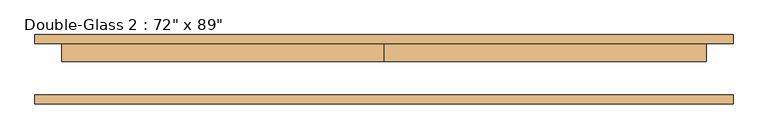
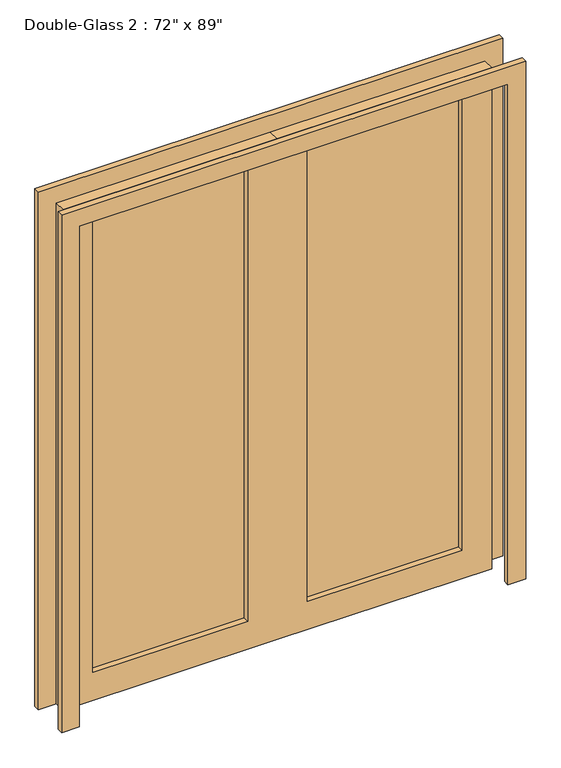
"""IFC4 building model written with IfcOpenShell, lengths in millimetres: door geometry."""

from ifc_helpers import new_model, si_unit, frame, origin, place, context, project, spatial, polyline, outline, extrude, source, transform, mapped, element, save


def door_20d24324(model_context):
    return source(origin(), model_context, "Body", "SweptSolid", [
        extrude(outline(polyline([(2260.6, 0.0), (2260.6, -914.4), (0.0, -914.4), (0.0, 0.0), (0.0, 914.4), (2260.6, 914.4), (2260.6, 0.0)]), holes=[polyline([(127.0, 787.4), (127.0, 127.0), (2184.4, 127.0), (2184.4, 787.4), (127.0, 787.4)]), polyline([(127.0, -787.4), (2184.4, -787.4), (2184.4, -127.0), (127.0, -127.0), (127.0, -787.4)])]), frame((0.0, 22.225, 0.0), z_axis=(0.0, 1.0, 0.0), x_axis=(0.0, 0.0, 1.0)), (0.0, 0.0, 1.0), 50.8),
        extrude(outline(polyline([(2260.6, -914.4), (2260.6, 914.4), (0.0, 914.4), (0.0, 990.6), (2336.8, 990.6), (2336.8, -990.6), (0.0, -990.6), (0.0, -914.4), (2260.6, -914.4)])), frame((0.0, -98.425, 0.0), z_axis=(0.0, 1.0, 0.0), x_axis=(0.0, 0.0, 1.0)), (0.0, 0.0, 1.0), 25.4),
        extrude(outline(polyline([(2260.6, -914.4), (2260.6, 914.4), (0.0, 914.4), (0.0, 990.6), (2336.8, 990.6), (2336.8, -990.6), (0.0, -990.6), (0.0, -914.4), (2260.6, -914.4)])), frame((0.0, 73.025, 0.0), z_axis=(0.0, 1.0, 0.0), x_axis=(0.0, 0.0, 1.0)), (0.0, 0.0, 1.0), 25.4),
        extrude(outline(polyline([(127.0, 53.975), (787.4, 53.975), (787.4, 47.625), (127.0, 47.625), (127.0, 53.975)])), frame((0.0, 0.0, 127.0), z_axis=(0.0, 0.0, 1.0), x_axis=(1.0, 0.0, 0.0)), (0.0, 0.0, 1.0), 2057.4),
        extrude(outline(polyline([(-787.4, 53.975), (-127.0, 53.975), (-127.0, 47.625), (-787.4, 47.625), (-787.4, 53.975)])), frame((0.0, 0.0, 127.0), z_axis=(0.0, 0.0, 1.0), x_axis=(1.0, 0.0, 0.0)), (0.0, 0.0, 1.0), 2057.4),
    ])


if __name__ == "__main__":
    model = new_model("IFC4")
    model_context = context("Model", 3, world=origin())
    ifc_project = project(units=[si_unit("LENGTHUNIT", "METRE", prefix="MILLI")], contexts=[model_context])
    site = spatial("IfcSite", under=ifc_project)
    building = spatial("IfcBuilding", under=site)
    placement = place(None, origin())
    door_shape = door_20d24324(model_context)
    element("IfcDoor", 1, ObjectType="Double-Glass 2 : 72\" x 89\"", at=placement, inside=building, context=model_context, shape_type="MappedRepresentation", body=[
        mapped(door_shape, transform((0.0, 0.0, 0.0), x_axis=(1.0, 0.0, 0.0), y_axis=(0.0, 1.0, 0.0), z_axis=(0.0, 0.0, 1.0))),
    ])
    save(model, "model.ifc")

# Revit data of these elements
# Type "Double-Glass 2 : 72\" x 89\""
#   Type Mark = "20"
#   Construction Type Id = "GSP4R"
#   Assembly Code = "C1020"
#   Analytic Construction = "1/8 in Pilkington single glazing"
#   Visual Light Transmittance = 0.9
#   Thickness = 0' - 2"
#   Solar Heat Gain Coefficient = 0.78
#   Heat Transfer Coefficient (U) = 3.6886 W/(m²·K)
#   Height = 7' - 5"
#   Muntin = 0' - 1"
#   Trim Projection Ext = 0' - 1"
#   Trim Projection Int = 0' - 1"
#   Trim Width = 0' - 3"
#   Width = 6' - 0"
#   Door Material = Aluminum
#   Frame Material = Aluminum
#   Thermal Resistance (R) = 0
#   Function = (empty or 0)
#   Wall Closure = (empty or 0)
# Element 1 (IfcDoor, "Double-Glass 2 : 72\" x 89\"")
#   Materials on its faces: "Aluminum", "Glass"
# Materials
#   "Aluminum": class "Metal", colour RGB 247 247 247, transparency 0, Description = "Aluminum 6061", Cost = 0
#   "Glass": class "Glass", colour RGB 218 227 224, transparency 0.85, Description = "Soda Lime Glass", Cost = 0
